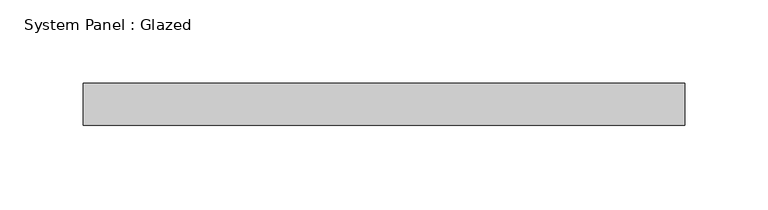
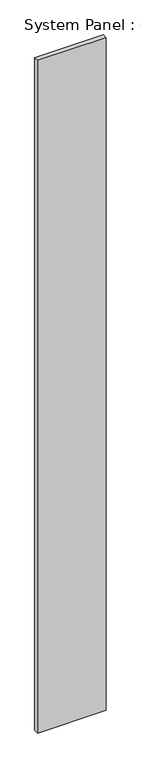
"""IFC4 building model written with IfcOpenShell, lengths in millimetres: plate geometry, System Panel : Glazed."""

import ifcopenshell
import ifcopenshell.guid

model = None  # the IFC model being written
_history = None  # IfcOwnerHistory: only IFC2X3 demands one
_inside = {}  # id of a spatial element -> (the spatial element, [elements in it])
_under = {}  # id of a project, library or spatial element -> (it, [spatial elements below it])
_declared = {}  # id of a project -> (the project, [libraries it declares])
_typed = {}  # id of a type object -> (the type object, [elements of that type])
_made_of = {}  # id of a material, layer set ... -> (it, [elements and type objects made of it])


def new_model(schema):
    """Start an empty IFC model of exactly this schema.

    Asked for "IFC4X3", IfcOpenShell would pick the latest addendum, in which some entities
    have other attributes; the version numbers below select the first issue.
    IFC2X3 requires an IfcOwnerHistory on every rooted entity: one is made here for all.
    """
    global model, _history
    if schema == "IFC4X3":
        model = ifcopenshell.file(schema_version=(4, 3, 0, 0))
    else:
        model = ifcopenshell.file(schema=schema)
    _inside.clear()
    _under.clear()
    _declared.clear()
    _typed.clear()
    _made_of.clear()
    _history = None
    if model.schema == "IFC2X3":
        org = make("IfcOrganization", Name="unknown")
        user = make(
            "IfcPersonAndOrganization",
            ThePerson=make("IfcPerson", FamilyName="unknown"),
            TheOrganization=org,
        )
        app = make(
            "IfcApplication",
            ApplicationDeveloper=org,
            Version="unknown",
            ApplicationFullName="unknown",
            ApplicationIdentifier="unknown",
        )
        _history = make(
            "IfcOwnerHistory",
            OwningUser=user,
            OwningApplication=app,
            ChangeAction="ADDED",
            CreationDate=0,
        )
    return model


def make(cls, **values):
    """One entity of the class cls with the attributes given. An attribute that is None is left unset."""
    return model.create_entity(
        cls, **{name: value for name, value in values.items() if value is not None}
    )


def rooted(cls, **values):
    """An entity with a GlobalId (a new one), such as an element, a storey or a relation."""
    return make(cls, GlobalId=ifcopenshell.guid.new(), OwnerHistory=_history, **values)


def si_unit(unit_type, name, prefix=None):
    """IfcSIUnit, for example si_unit("LENGTHUNIT", "METRE", prefix="MILLI")."""
    return make("IfcSIUnit", UnitType=unit_type, Prefix=prefix, Name=name)


def assignment(units):
    """IfcUnitAssignment: the units of a project."""
    return None if units is None else make("IfcUnitAssignment", Units=units)


def point(xyz):
    """IfcCartesianPoint."""
    return None if xyz is None else make("IfcCartesianPoint", Coordinates=xyz)


def direction(xyz):
    """IfcDirection."""
    return None if xyz is None else make("IfcDirection", DirectionRatios=xyz)


def frame(location, z_axis=None, x_axis=None):
    """IfcAxis2Placement3D, a coordinate frame: its origin and axes. An axis left out is left unset."""
    return make(
        "IfcAxis2Placement3D",
        Location=point(location),
        Axis=direction(z_axis),
        RefDirection=direction(x_axis),
    )


def origin():
    """The frame at (0, 0, 0) with its axes left unset."""
    return frame((0.0, 0.0, 0.0))


def origin_with_axes():
    """The frame at (0, 0, 0) with the z axis (0, 0, 1) and the x axis (1, 0, 0) written out."""
    return frame((0.0, 0.0, 0.0), z_axis=(0.0, 0.0, 1.0), x_axis=(1.0, 0.0, 0.0))


def place(relative_to, where):
    """IfcLocalPlacement: puts the frame where relative to a parent placement (None: the world)."""
    return make(
        "IfcLocalPlacement", PlacementRelTo=relative_to, RelativePlacement=where
    )


def context(
    kind, dimensions, precision=None, world=None, true_north=None, identifier=None
):
    """IfcGeometricRepresentationContext, for example the 3D "Model" context."""
    return make(
        "IfcGeometricRepresentationContext",
        ContextIdentifier=identifier,
        ContextType=kind,
        CoordinateSpaceDimension=dimensions,
        Precision=precision,
        WorldCoordinateSystem=world,
        TrueNorth=true_north,
    )


def project(units=None, contexts=None):
    """IfcProject with its units and contexts."""
    return rooted(
        "IfcProject",
        Name="project",
        RepresentationContexts=contexts,
        UnitsInContext=assignment(units),
    )


def spatial(cls, under=None, at=None, **own):
    """A site, building, storey or space (cls), placed at a placement, below another one or the project."""
    s = rooted(cls, ObjectPlacement=at, **own)
    if under is not None:
        _under.setdefault(under.id(), (under, []))[1].append(s)
    return s


def polyline(points):
    """IfcPolyline through the points."""
    return make("IfcPolyline", Points=[point(p) for p in points])


def outline(outer, holes=None, kind="AREA"):
    """IfcArbitraryClosedProfileDef: a profile drawn as a closed curve; with holes, ...WithVoids."""
    if holes is None:
        return make("IfcArbitraryClosedProfileDef", ProfileType=kind, OuterCurve=outer)
    return make(
        "IfcArbitraryProfileDefWithVoids",
        ProfileType=kind,
        OuterCurve=outer,
        InnerCurves=holes,
    )


def extrude(swept, where, along, depth):
    """IfcExtrudedAreaSolid: the profile swept, set in the frame where, extruded along a direction by depth."""
    return make(
        "IfcExtrudedAreaSolid",
        SweptArea=swept,
        Position=where,
        ExtrudedDirection=direction(along),
        Depth=depth,
    )


def shape(context_of_items, identifier, shape_type, items):
    """IfcShapeRepresentation: the items that make up one representation, for example the "Body"."""
    return make(
        "IfcShapeRepresentation",
        ContextOfItems=context_of_items,
        RepresentationIdentifier=identifier,
        RepresentationType=shape_type,
        Items=items,
    )


def source(mapping_origin, context_of_items, identifier, shape_type, items):
    """IfcRepresentationMap: a shape defined once, which mapped items show again and again."""
    return make(
        "IfcRepresentationMap",
        MappingOrigin=mapping_origin,
        MappedRepresentation=shape(context_of_items, identifier, shape_type, items),
    )


def transform(
    local_origin,
    x_axis=None,
    y_axis=None,
    z_axis=None,
    scale=None,
    scale2=None,
    scale3=None,
    uniform=True,
):
    """IfcCartesianTransformationOperator3D, or its non-uniform kind. x_axis, y_axis, z_axis: its Axis1, 2, 3."""
    if uniform:
        return make(
            "IfcCartesianTransformationOperator3D",
            Axis1=direction(x_axis),
            Axis2=direction(y_axis),
            LocalOrigin=point(local_origin),
            Scale=scale,
            Axis3=direction(z_axis),
        )
    return make(
        "IfcCartesianTransformationOperator3DnonUniform",
        Axis1=direction(x_axis),
        Axis2=direction(y_axis),
        LocalOrigin=point(local_origin),
        Scale=scale,
        Axis3=direction(z_axis),
        Scale2=scale2,
        Scale3=scale3,
    )


def mapped(mapping_source, mapping_target):
    """IfcMappedItem: shows the shape of a source again, moved by a transform."""
    return make(
        "IfcMappedItem", MappingSource=mapping_source, MappingTarget=mapping_target
    )


def made_of(thing, what):
    """Note that an element or type object is made of a material, layer set ...; save() writes the relation."""
    if what is not None:
        _made_of.setdefault(what.id(), (what, []))[1].append(thing)
    return thing


def element(
    cls,
    number,
    at=None,
    inside=None,
    cuts=None,
    type_object=None,
    material=None,
    context=None,
    identifier="Body",
    shape_type=None,
    held_by="IfcProductDefinitionShape",
    body=None,
    shapes=None,
    **own,
):
    """One element of the class cls, such as IfcWall. Its Tag is "e" and its number.

    at: its placement. inside: the storey or other place that contains it. cuts: it is an
    opening in that element (IfcRelVoidsElement). A single representation is given by context,
    identifier, shape_type and body (its items); several are given by shapes. held_by: the class
    of the entity that holds the representations. save() writes the other relations.
    """
    e = rooted(cls, Tag="e%d" % number, ObjectPlacement=at, **own)
    if body is not None:
        shapes = [shape(context, identifier, shape_type, body)]
    if shapes is not None:
        e.Representation = make(held_by, Representations=shapes)
    if inside is not None:
        _inside.setdefault(inside.id(), (inside, []))[1].append(e)
    if cuts is not None:
        rooted(
            "IfcRelVoidsElement", RelatingBuildingElement=cuts, RelatedOpeningElement=e
        )
    if type_object is not None:
        _typed.setdefault(type_object.id(), (type_object, []))[1].append(e)
    return made_of(e, material)


def aggregate(whole, parts):
    """IfcRelAggregates: a whole, such as a stair, and the parts it consists of."""
    return rooted("IfcRelAggregates", RelatingObject=whole, RelatedObjects=parts)


def save(model, path):
    """Write the relations noted so far, then the file.

    IfcRelAggregates (storeys below a building ...), IfcRelContainedInSpatialStructure (elements
    in a storey), IfcRelDefinesByType, IfcRelAssociatesMaterial and IfcRelDeclares: one each for
    every whole, place, type object, material and project.
    """
    for whole, parts in _under.values():
        aggregate(whole, parts)
    for where, things in _inside.values():
        rooted(
            "IfcRelContainedInSpatialStructure",
            RelatedElements=things,
            RelatingStructure=where,
        )
    for kind, things in _typed.values():
        rooted("IfcRelDefinesByType", RelatedObjects=things, RelatingType=kind)
    for what, things in _made_of.values():
        rooted("IfcRelAssociatesMaterial", RelatedObjects=things, RelatingMaterial=what)
    for by, libraries in _declared.values():
        rooted("IfcRelDeclares", RelatingContext=by, RelatedDefinitions=libraries)
    model.write(path)


def system_panel_glazed_032e4dab(model_context):
    return source(origin(), model_context, "Body", "SweptSolid", [
        extrude(outline(polyline([(180.975, 19.05), (-180.975, 19.05), (-180.975, 44.45), (180.975, 44.45), (180.975, 19.05)])), origin_with_axes(), (0.0, 0.0, 1.0), 3746.5),
    ])


if __name__ == "__main__":
    model = new_model("IFC4")
    model_context = context("Model", 3, world=origin())
    ifc_project = project(units=[si_unit("LENGTHUNIT", "METRE", prefix="MILLI")], contexts=[model_context])
    site = spatial("IfcSite", under=ifc_project)
    building = spatial("IfcBuilding", under=site)
    placement = place(None, origin())
    system_panel_glazed_shape = system_panel_glazed_032e4dab(model_context)
    element("IfcPlate", 1, ObjectType="System Panel : Glazed", at=placement, inside=building, context=model_context, shape_type="MappedRepresentation", body=[
        mapped(system_panel_glazed_shape, transform((0.0, 0.0, 0.0), x_axis=(1.0, 0.0, 0.0), y_axis=(0.0, 1.0, 0.0), z_axis=(0.0, 0.0, 1.0))),
    ])
    save(model, "model.ifc")

# Revit data of these elements
# Type "System Panel : Glazed"
#   Construction Type Id = "GSP4R"
#   Analytic Construction = "1/8 in Pilkington single glazing"
#   Visual Light Transmittance = 0.9
#   Solar Heat Gain Coefficient = 0.86
#   Heat Transfer Coefficient (U) = 1.18115 BTU/(h·ft²·°F)
#   Define Thermal Properties by = 1
# Element 1 (IfcPlate, "System Panel : Glazed")
#   Materials on its faces: "Glass"
# Materials
#   "Glass": class "Glass", colour RGB 0 128 192, transparency 0.75, Description = "Soda Lime Glass", Cost = 0
